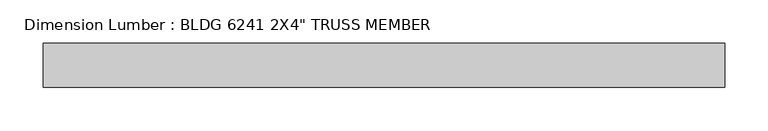
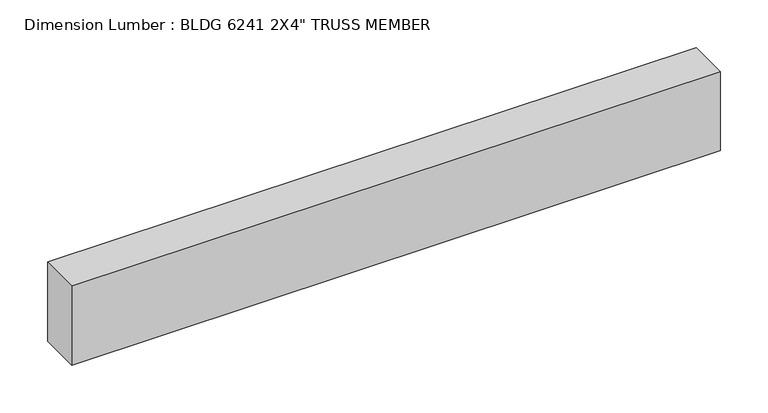
"""IFC4 building model written with IfcOpenShell, lengths in millimetres: beam geometry."""

from ifc_helpers import new_model, si_unit, frame, origin, place, context, project, spatial, polyline, outline, extrude, source, transform, mapped, element, save


def beam_7745fe0f(model_context):
    return source(origin(), model_context, "Body", "SweptSolid", [
        extrude(outline(polyline([(393.7, 25.4), (393.7, -25.4), (-393.7, -25.4), (-393.7, 25.4), (393.7, 25.4)])), frame((0.0, 0.0, -50.8), z_axis=(0.0, 0.0, 1.0), x_axis=(1.0, 0.0, 0.0)), (0.0, 0.0, 1.0), 101.6),
    ])


if __name__ == "__main__":
    model = new_model("IFC4")
    model_context = context("Model", 3, world=origin())
    ifc_project = project(units=[si_unit("LENGTHUNIT", "METRE", prefix="MILLI")], contexts=[model_context])
    site = spatial("IfcSite", under=ifc_project)
    building = spatial("IfcBuilding", under=site)
    placement = place(None, origin())
    beam_shape = beam_7745fe0f(model_context)
    element("IfcBeam", 1, ObjectType="Dimension Lumber : BLDG 6241 2X4\" TRUSS MEMBER", at=placement, inside=building, context=model_context, shape_type="MappedRepresentation", body=[
        mapped(beam_shape, transform((0.0, 0.0, 0.0), x_axis=(1.0, 0.0, 0.0), y_axis=(0.0, 1.0, 0.0), z_axis=(0.0, 0.0, 1.0))),
    ])
    save(model, "model.ifc")

# Revit data of these elements
# Type "Dimension Lumber : BLDG 6241 2X4\" TRUSS MEMBER"
#   Assembly Code = "B10"
#   A = 0.273472 SF
#   Length [instance default] = 5' - 0"
#   b = 0' - 2"
#   d = 0' - 4"
#   Structural Material [instance default] = Softwood, Lumber
# Element 1 (IfcBeam, "Dimension Lumber : BLDG 6241 2X4\" TRUSS MEMBER")
#   Materials on its faces: "Softwood, Lumber"
# Materials
#   "Softwood, Lumber": class "Wood", colour RGB 223 192 134, transparency 0, Description = "Pinus Echinata", Cost = 0
